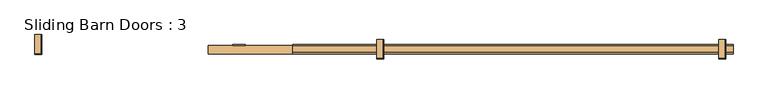
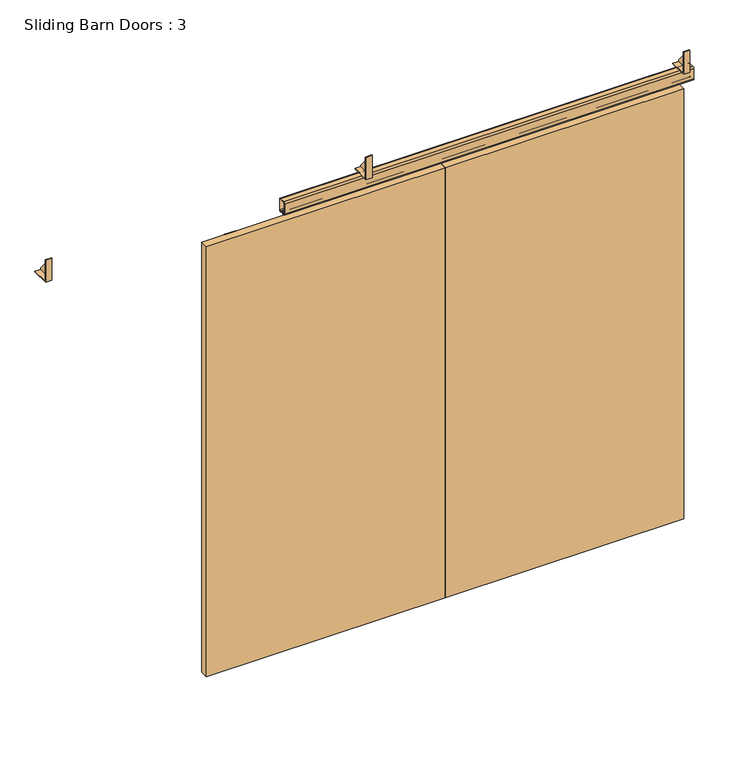
"""IFC4 building model written with IfcOpenShell, lengths in millimetres: door geometry, Sliding Barn Doors : 3."""

import ifcopenshell
import ifcopenshell.guid

model = None  # the IFC model being written
_history = None  # IfcOwnerHistory: only IFC2X3 demands one
_inside = {}  # id of a spatial element -> (the spatial element, [elements in it])
_under = {}  # id of a project, library or spatial element -> (it, [spatial elements below it])
_declared = {}  # id of a project -> (the project, [libraries it declares])
_typed = {}  # id of a type object -> (the type object, [elements of that type])
_made_of = {}  # id of a material, layer set ... -> (it, [elements and type objects made of it])


def new_model(schema):
    """Start an empty IFC model of exactly this schema.

    Asked for "IFC4X3", IfcOpenShell would pick the latest addendum, in which some entities
    have other attributes; the version numbers below select the first issue.
    IFC2X3 requires an IfcOwnerHistory on every rooted entity: one is made here for all.
    """
    global model, _history
    if schema == "IFC4X3":
        model = ifcopenshell.file(schema_version=(4, 3, 0, 0))
    else:
        model = ifcopenshell.file(schema=schema)
    _inside.clear()
    _under.clear()
    _declared.clear()
    _typed.clear()
    _made_of.clear()
    _history = None
    if model.schema == "IFC2X3":
        org = make("IfcOrganization", Name="unknown")
        user = make(
            "IfcPersonAndOrganization",
            ThePerson=make("IfcPerson", FamilyName="unknown"),
            TheOrganization=org,
        )
        app = make(
            "IfcApplication",
            ApplicationDeveloper=org,
            Version="unknown",
            ApplicationFullName="unknown",
            ApplicationIdentifier="unknown",
        )
        _history = make(
            "IfcOwnerHistory",
            OwningUser=user,
            OwningApplication=app,
            ChangeAction="ADDED",
            CreationDate=0,
        )
    return model


def make(cls, **values):
    """One entity of the class cls with the attributes given. An attribute that is None is left unset."""
    return model.create_entity(
        cls, **{name: value for name, value in values.items() if value is not None}
    )


def rooted(cls, **values):
    """An entity with a GlobalId (a new one), such as an element, a storey or a relation."""
    return make(cls, GlobalId=ifcopenshell.guid.new(), OwnerHistory=_history, **values)


def si_unit(unit_type, name, prefix=None):
    """IfcSIUnit, for example si_unit("LENGTHUNIT", "METRE", prefix="MILLI")."""
    return make("IfcSIUnit", UnitType=unit_type, Prefix=prefix, Name=name)


def assignment(units):
    """IfcUnitAssignment: the units of a project."""
    return None if units is None else make("IfcUnitAssignment", Units=units)


def point(xyz):
    """IfcCartesianPoint."""
    return None if xyz is None else make("IfcCartesianPoint", Coordinates=xyz)


def direction(xyz):
    """IfcDirection."""
    return None if xyz is None else make("IfcDirection", DirectionRatios=xyz)


def frame(location, z_axis=None, x_axis=None):
    """IfcAxis2Placement3D, a coordinate frame: its origin and axes. An axis left out is left unset."""
    return make(
        "IfcAxis2Placement3D",
        Location=point(location),
        Axis=direction(z_axis),
        RefDirection=direction(x_axis),
    )


def frame_2d(location, x_axis=None):
    """IfcAxis2Placement2D, a coordinate frame in the plane: its origin and x axis."""
    return make(
        "IfcAxis2Placement2D", Location=point(location), RefDirection=direction(x_axis)
    )


def origin():
    """The frame at (0, 0, 0) with its axes left unset."""
    return frame((0.0, 0.0, 0.0))


def place(relative_to, where):
    """IfcLocalPlacement: puts the frame where relative to a parent placement (None: the world)."""
    return make(
        "IfcLocalPlacement", PlacementRelTo=relative_to, RelativePlacement=where
    )


def context(
    kind, dimensions, precision=None, world=None, true_north=None, identifier=None
):
    """IfcGeometricRepresentationContext, for example the 3D "Model" context."""
    return make(
        "IfcGeometricRepresentationContext",
        ContextIdentifier=identifier,
        ContextType=kind,
        CoordinateSpaceDimension=dimensions,
        Precision=precision,
        WorldCoordinateSystem=world,
        TrueNorth=true_north,
    )


def project(units=None, contexts=None):
    """IfcProject with its units and contexts."""
    return rooted(
        "IfcProject",
        Name="project",
        RepresentationContexts=contexts,
        UnitsInContext=assignment(units),
    )


def spatial(cls, under=None, at=None, **own):
    """A site, building, storey or space (cls), placed at a placement, below another one or the project."""
    s = rooted(cls, ObjectPlacement=at, **own)
    if under is not None:
        _under.setdefault(under.id(), (under, []))[1].append(s)
    return s


def polyline(points):
    """IfcPolyline through the points."""
    return make("IfcPolyline", Points=[point(p) for p in points])


def circle_curve(where, radius):
    """IfcCircle in the frame where."""
    return make("IfcCircle", Position=where, Radius=radius)


def trimmed(basis, trim1, trim2, sense, master):
    """IfcTrimmedCurve: the piece of a basis curve between two trims."""
    return make(
        "IfcTrimmedCurve",
        BasisCurve=basis,
        Trim1=trim1,
        Trim2=trim2,
        SenseAgreement=sense,
        MasterRepresentation=master,
    )


def segment(curve, same_sense, transition):
    """IfcCompositeCurveSegment."""
    return make(
        "IfcCompositeCurveSegment",
        Transition=transition,
        SameSense=same_sense,
        ParentCurve=curve,
    )


def composite_curve(segments, self_intersect=None):
    """IfcCompositeCurve: segments joined end to end."""
    return make("IfcCompositeCurve", Segments=segments, SelfIntersect=self_intersect)


def outline(outer, holes=None, kind="AREA"):
    """IfcArbitraryClosedProfileDef: a profile drawn as a closed curve; with holes, ...WithVoids."""
    if holes is None:
        return make("IfcArbitraryClosedProfileDef", ProfileType=kind, OuterCurve=outer)
    return make(
        "IfcArbitraryProfileDefWithVoids",
        ProfileType=kind,
        OuterCurve=outer,
        InnerCurves=holes,
    )


def extrude(swept, where, along, depth):
    """IfcExtrudedAreaSolid: the profile swept, set in the frame where, extruded along a direction by depth."""
    return make(
        "IfcExtrudedAreaSolid",
        SweptArea=swept,
        Position=where,
        ExtrudedDirection=direction(along),
        Depth=depth,
    )


def shape(context_of_items, identifier, shape_type, items):
    """IfcShapeRepresentation: the items that make up one representation, for example the "Body"."""
    return make(
        "IfcShapeRepresentation",
        ContextOfItems=context_of_items,
        RepresentationIdentifier=identifier,
        RepresentationType=shape_type,
        Items=items,
    )


def source(mapping_origin, context_of_items, identifier, shape_type, items):
    """IfcRepresentationMap: a shape defined once, which mapped items show again and again."""
    return make(
        "IfcRepresentationMap",
        MappingOrigin=mapping_origin,
        MappedRepresentation=shape(context_of_items, identifier, shape_type, items),
    )


def transform(
    local_origin,
    x_axis=None,
    y_axis=None,
    z_axis=None,
    scale=None,
    scale2=None,
    scale3=None,
    uniform=True,
):
    """IfcCartesianTransformationOperator3D, or its non-uniform kind. x_axis, y_axis, z_axis: its Axis1, 2, 3."""
    if uniform:
        return make(
            "IfcCartesianTransformationOperator3D",
            Axis1=direction(x_axis),
            Axis2=direction(y_axis),
            LocalOrigin=point(local_origin),
            Scale=scale,
            Axis3=direction(z_axis),
        )
    return make(
        "IfcCartesianTransformationOperator3DnonUniform",
        Axis1=direction(x_axis),
        Axis2=direction(y_axis),
        LocalOrigin=point(local_origin),
        Scale=scale,
        Axis3=direction(z_axis),
        Scale2=scale2,
        Scale3=scale3,
    )


def mapped(mapping_source, mapping_target):
    """IfcMappedItem: shows the shape of a source again, moved by a transform."""
    return make(
        "IfcMappedItem", MappingSource=mapping_source, MappingTarget=mapping_target
    )


def made_of(thing, what):
    """Note that an element or type object is made of a material, layer set ...; save() writes the relation."""
    if what is not None:
        _made_of.setdefault(what.id(), (what, []))[1].append(thing)
    return thing


def element(
    cls,
    number,
    at=None,
    inside=None,
    cuts=None,
    type_object=None,
    material=None,
    context=None,
    identifier="Body",
    shape_type=None,
    held_by="IfcProductDefinitionShape",
    body=None,
    shapes=None,
    **own,
):
    """One element of the class cls, such as IfcWall. Its Tag is "e" and its number.

    at: its placement. inside: the storey or other place that contains it. cuts: it is an
    opening in that element (IfcRelVoidsElement). A single representation is given by context,
    identifier, shape_type and body (its items); several are given by shapes. held_by: the class
    of the entity that holds the representations. save() writes the other relations.
    """
    e = rooted(cls, Tag="e%d" % number, ObjectPlacement=at, **own)
    if body is not None:
        shapes = [shape(context, identifier, shape_type, body)]
    if shapes is not None:
        e.Representation = make(held_by, Representations=shapes)
    if inside is not None:
        _inside.setdefault(inside.id(), (inside, []))[1].append(e)
    if cuts is not None:
        rooted(
            "IfcRelVoidsElement", RelatingBuildingElement=cuts, RelatedOpeningElement=e
        )
    if type_object is not None:
        _typed.setdefault(type_object.id(), (type_object, []))[1].append(e)
    return made_of(e, material)


def aggregate(whole, parts):
    """IfcRelAggregates: a whole, such as a stair, and the parts it consists of."""
    return rooted("IfcRelAggregates", RelatingObject=whole, RelatedObjects=parts)


def save(model, path):
    """Write the relations noted so far, then the file.

    IfcRelAggregates (storeys below a building ...), IfcRelContainedInSpatialStructure (elements
    in a storey), IfcRelDefinesByType, IfcRelAssociatesMaterial and IfcRelDeclares: one each for
    every whole, place, type object, material and project.
    """
    for whole, parts in _under.values():
        aggregate(whole, parts)
    for where, things in _inside.values():
        rooted(
            "IfcRelContainedInSpatialStructure",
            RelatedElements=things,
            RelatingStructure=where,
        )
    for kind, things in _typed.values():
        rooted("IfcRelDefinesByType", RelatedObjects=things, RelatingType=kind)
    for what, things in _made_of.values():
        rooted("IfcRelAssociatesMaterial", RelatedObjects=things, RelatingMaterial=what)
    for by, libraries in _declared.values():
        rooted("IfcRelDeclares", RelatingContext=by, RelatedDefinitions=libraries)
    model.write(path)


def sliding_barn_doors_3_ff6fe0db(model_context):
    return source(origin(), model_context, "Body", "SweptSolid", [
        extrude(outline(polyline([(158.75, 2152.65), (158.75, 2146.3), (79.375, 2146.3), (79.375, 2247.773), (158.75, 2152.65)])), frame((-1635.1746094, 0.0, 0.0), z_axis=(1.0, 0.0, 0.0), x_axis=(0.0, 1.0, 0.0)), (0.0, 0.0, 1.0), 3.175),
        extrude(outline(polyline([(76.2, 2143.125), (76.2, 2247.773), (79.375, 2247.773), (79.375, 2146.3), (158.75, 2146.3), (158.75, 2143.125), (76.2, 2143.125)])), frame((-1660.4753906, 0.0, 0.0), z_axis=(1.0, 0.0, 0.0), x_axis=(0.0, 1.0, 0.0)), (0.0, 0.0, 1.0), 28.4757812),
        extrude(outline(polyline([(139.7, 2152.65), (139.7, 2146.3), (60.325, 2146.3), (60.325, 2247.773), (139.7, 2152.65)])), frame((-215.1558594, 0.0, 0.0), z_axis=(1.0, 0.0, 0.0), x_axis=(0.0, 1.0, 0.0)), (0.0, 0.0, 1.0), 3.175),
        extrude(outline(polyline([(57.15, 2143.125), (57.15, 2247.773), (60.325, 2247.773), (60.325, 2146.3), (139.7, 2146.3), (139.7, 2143.125), (57.15, 2143.125)])), frame((-240.4566406, 0.0, 0.0), z_axis=(1.0, 0.0, 0.0), x_axis=(0.0, 1.0, 0.0)), (0.0, 0.0, 1.0), 28.4757812),
        extrude(outline(polyline([(139.7, 2152.65), (139.7, 2146.3), (60.325, 2146.3), (60.325, 2247.773), (139.7, 2152.65)])), frame((1204.8628906, 0.0, 0.0), z_axis=(1.0, 0.0, 0.0), x_axis=(0.0, 1.0, 0.0)), (0.0, 0.0, 1.0), 3.175),
        extrude(outline(polyline([(57.15, 2143.125), (57.15, 2247.773), (60.325, 2247.773), (60.325, 2146.3), (139.7, 2146.3), (139.7, 2143.125), (57.15, 2143.125)])), frame((1179.5621094, 0.0, 0.0), z_axis=(1.0, 0.0, 0.0), x_axis=(0.0, 1.0, 0.0)), (0.0, 0.0, 1.0), 28.4757812),
        extrude(outline(polyline([(-838.454, 117.475), (-787.146, 117.475), (-787.146, 114.3), (-838.454, 114.3), (-838.454, 117.475)])), frame((0.0, 0.0, 1889.252), z_axis=(0.0, 0.0, 1.0), x_axis=(1.0, 0.0, 0.0)), (0.0, 0.0, 1.0), 168.148),
        extrude(outline(polyline([(-25.654, 117.475), (25.654, 117.475), (25.654, 114.3), (-25.654, 114.3), (-25.654, 117.475)])), frame((0.0, 0.0, 1889.252), z_axis=(0.0, 0.0, 1.0), x_axis=(1.0, 0.0, 0.0)), (0.0, 0.0, 1.0), 168.148),
        extrude(outline(polyline([(228.346, 117.475), (279.654, 117.475), (279.654, 114.3), (228.346, 114.3), (228.346, 117.475)])), frame((0.0, 0.0, 1889.252), z_axis=(0.0, 0.0, 1.0), x_axis=(1.0, 0.0, 0.0)), (0.0, 0.0, 1.0), 168.148),
        extrude(outline(polyline([(1041.146, 117.475), (1092.454, 117.475), (1092.454, 114.3), (1041.146, 114.3), (1041.146, 117.475)])), frame((0.0, 0.0, 1889.252), z_axis=(0.0, 0.0, 1.0), x_axis=(1.0, 0.0, 0.0)), (0.0, 0.0, 1.0), 168.148),
        extrude(outline(polyline([(-939.8, 114.3), (127.0, 114.3), (127.0, 79.375), (-939.8, 79.375), (-939.8, 114.3)])), frame((0.0, 0.0, 25.4), z_axis=(0.0, 0.0, 1.0), x_axis=(1.0, 0.0, 0.0)), (0.0, 0.0, 1.0), 2032.0),
        extrude(outline(polyline([(127.0, 114.3), (1193.8, 114.3), (1193.8, 79.375), (127.0, 79.375), (127.0, 114.3)])), frame((0.0, 0.0, 25.4), z_axis=(0.0, 0.0, 1.0), x_axis=(1.0, 0.0, 0.0)), (0.0, 0.0, 1.0), 2032.0),
        extrude(outline(composite_curve([segment(polyline([(85.725, 2143.125), (111.252, 2143.125)]), True, "CONTINUOUS"), segment(trimmed(circle_curve(frame_2d((111.252, 2136.775)), 6.35), [point((111.252, 2143.125))], [point((117.602, 2136.775))], False, "CARTESIAN"), True, "CONTINUOUS"), segment(polyline([(117.602, 2136.775), (117.602, 2088.515)]), True, "CONTINUOUS"), segment(trimmed(circle_curve(frame_2d((111.252, 2088.515)), 6.35), [point((117.602, 2088.515))], [point((111.252, 2082.165))], False, "CARTESIAN"), True, "CONTINUOUS"), segment(polyline([(111.252, 2082.165), (105.8433147, 2082.165)]), True, "CONTINUOUS"), segment(trimmed(circle_curve(frame_2d((105.8433147, 2083.7525)), 1.5875), [point((105.8433147, 2082.165))], [point((104.2849816, 2083.4495907))], False, "CARTESIAN"), True, "CONTINUOUS"), segment(polyline([(104.2849816, 2083.4495907), (102.8594659, 2090.7832331), (104.3756029, 2090.7832331), (105.7615251, 2083.6532812), (111.252, 2083.6532812)]), True, "CONTINUOUS"), segment(trimmed(circle_curve(frame_2d((111.252, 2088.515)), 4.8617187), [point((111.252, 2083.6532812))], [point((116.1137188, 2088.515))], True, "CARTESIAN"), True, "CONTINUOUS"), segment(polyline([(116.1137188, 2088.515), (116.1137188, 2136.775)]), True, "CONTINUOUS"), segment(trimmed(circle_curve(frame_2d((111.252, 2136.775)), 4.8617187), [point((116.1137188, 2136.775))], [point((111.252, 2141.6367187))], True, "CARTESIAN"), True, "CONTINUOUS"), segment(polyline([(111.252, 2141.6367187), (85.725, 2141.6367187)]), True, "CONTINUOUS"), segment(trimmed(circle_curve(frame_2d((85.725, 2136.775)), 4.8617187), [point((85.725, 2141.6367187))], [point((80.8632813, 2136.775))], True, "CARTESIAN"), True, "CONTINUOUS"), segment(polyline([(80.8632813, 2136.775), (80.8632813, 2088.515)]), True, "CONTINUOUS"), segment(trimmed(circle_curve(frame_2d((85.725, 2088.515)), 4.8617187), [point((80.8632813, 2088.515))], [point((85.725, 2083.6532812))], True, "CARTESIAN"), True, "CONTINUOUS"), segment(polyline([(85.725, 2083.6532812), (91.2154749, 2083.6532812), (92.6013971, 2090.7832331), (94.1175341, 2090.7832331), (92.6920184, 2083.4495907)]), True, "CONTINUOUS"), segment(trimmed(circle_curve(frame_2d((91.1336853, 2083.7525)), 1.5875), [point((92.6920184, 2083.4495907))], [point((91.1336853, 2082.165))], False, "CARTESIAN"), True, "CONTINUOUS"), segment(polyline([(91.1336853, 2082.165), (85.725, 2082.165)]), True, "CONTINUOUS"), segment(trimmed(circle_curve(frame_2d((85.725, 2088.515)), 6.35), [point((85.725, 2082.165))], [point((79.375, 2088.515))], False, "CARTESIAN"), True, "CONTINUOUS"), segment(polyline([(79.375, 2088.515), (79.375, 2136.775)]), True, "CONTINUOUS"), segment(trimmed(circle_curve(frame_2d((85.725, 2136.775)), 6.35), [point((79.375, 2136.775))], [point((85.725, 2143.125))], False, "CARTESIAN"), True, "CONTINUOUS")], self_intersect=False)), frame((-590.55, 0.0, 0.0), z_axis=(1.0, 0.0, 0.0), x_axis=(0.0, 1.0, 0.0)), (0.0, 0.0, 1.0), 1828.8),
    ])


if __name__ == "__main__":
    model = new_model("IFC4")
    model_context = context("Model", 3, world=origin())
    ifc_project = project(units=[si_unit("LENGTHUNIT", "METRE", prefix="MILLI")], contexts=[model_context])
    site = spatial("IfcSite", under=ifc_project)
    building = spatial("IfcBuilding", under=site)
    placement = place(None, origin())
    sliding_barn_doors_3_shape = sliding_barn_doors_3_ff6fe0db(model_context)
    element("IfcDoor", 1, ObjectType="Sliding Barn Doors : 3", at=placement, inside=building, context=model_context, shape_type="MappedRepresentation", body=[
        mapped(sliding_barn_doors_3_shape, transform((0.0, 0.0, 0.0), x_axis=(1.0, 0.0, 0.0), y_axis=(0.0, 1.0, 0.0), z_axis=(0.0, 0.0, 1.0))),
    ])
    save(model, "model.ifc")

# Revit data of these elements
# Type "Sliding Barn Doors : 3"
#   Type Mark = "43"
#   Analytic Construction = "<None>"
#   rail_overlap_left = 0' - 3 3/4"
#   rail_length = 6' - 0"
#   overlap_left = 0' - 2"
#   overlap = 0' - 0"
#   bracket_right = 1' - 7 13/16"
#   bracket_left = 0' - 2"
#   Thickness = 0' - 1 3/8"
#   Panel Width = 3' - 6"
#   Panel Height = 6' - 8"
#   Gap 2 = 0' - 0 1/2"
#   Gap 1 = 0' - 0 7/8"
#   Frame Projection Ext. = 0' - 1"
#   Frame Projection Int. = 0' - 1"
#   Frame Width = 0' - 3"
#   Height = 6' - 5 3/8"
#   Width = 7' - 6"
#   Bracket_offset = 0' - 5"
#   Door_4 = no
#   Door_3 = no
#   Hardware Material = Metal - Aluminum
#   Door Material = Closet_1
#   Function = (empty or 0)
#   Wall Closure = (empty or 0)
# Element 1 (IfcDoor, "Sliding Barn Doors : 3")
#   Materials on its faces: "Metal - Aluminum", "Closet_1"
# Materials
#   "Metal - Aluminum": class "Metal", colour RGB 247 247 247, transparency 0
#   "Closet_1": class "Paint", colour RGB 58 62 47, transparency 0, Cost = 0
